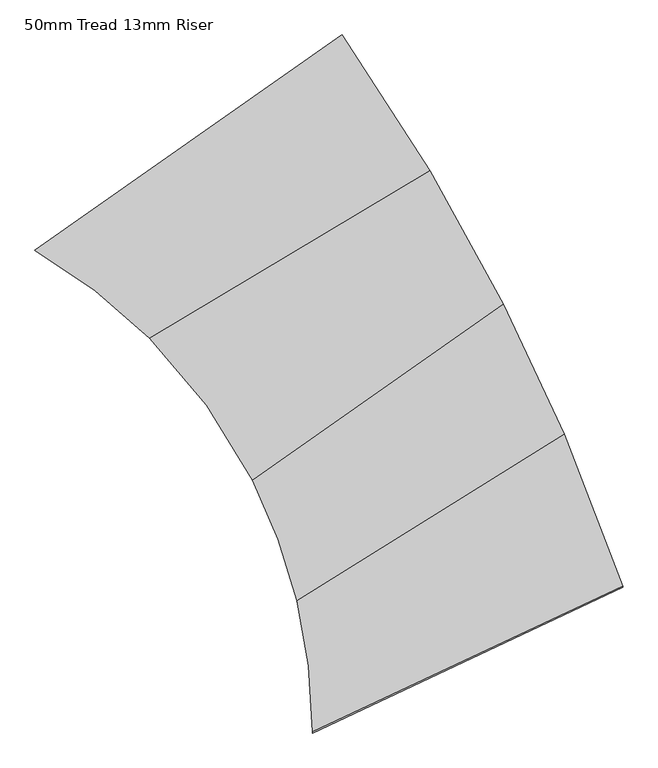
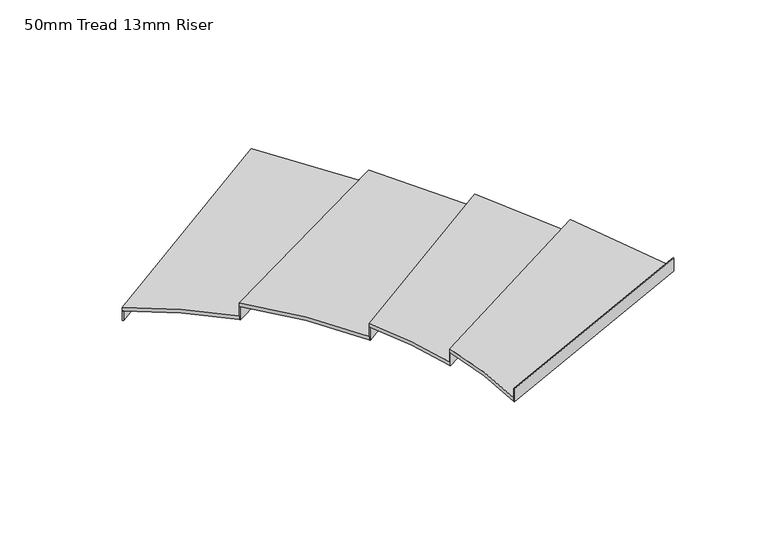
"""IFC4 building model written with IfcOpenShell, lengths in millimetres: stair flight geometry, 50mm Tread 13mm Riser."""

from ifc_helpers import new_model, si_unit, point, frame, frame_2d, origin, place, context, project, spatial, polyline, circle_curve, trimmed, segment, composite_curve, outline, extrude, source, transform, mapped, element, save


def stair_flight_50mm_tread_13mm_riser_794cdd2d(model_context):
    return source(origin(), model_context, "Body", "SweptSolid", [
        extrude(outline(composite_curve([segment(trimmed(circle_curve(frame_2d((18979.6163047, 39173.0351392)), 5303.3008589), [point((21646.6672, 43756.9024498))], [point((21634.7503997, 43763.8153492))], True, "CARTESIAN"), True, "CONTINUOUS"), segment(polyline([(21634.7503997, 43763.8153492), (24564.2523191, 45816.6486415)]), True, "CONTINUOUS"), segment(trimmed(circle_curve(frame_2d((7249.7804154, 33683.622161)), 21142.4045199), [point((24564.2523191, 45816.6486415))], [point((24571.4226886, 45806.4097053))], False, "CARTESIAN"), True, "CONTINUOUS"), segment(polyline([(24571.4226886, 45806.4097053), (21646.6672, 43756.9024498)]), True, "CONTINUOUS")], self_intersect=False)), frame((0.0, 0.0, 12000.0), z_axis=(0.0, 0.0, 1.0), x_axis=(1.0, 0.0, 0.0)), (0.0, 0.0, 1.0), 136.0465116),
        extrude(outline(composite_curve([segment(polyline([(25404.2827089, 44519.45694), (22729.6163047, 42923.0351392)]), True, "CONTINUOUS"), segment(trimmed(circle_curve(frame_2d((18979.6163047, 39173.0351392)), 5303.3008589), [point((22729.6163047, 42923.0351392))], [point((21634.7503997, 43763.8153492))], True, "CARTESIAN"), True, "CONTINUOUS"), segment(polyline([(21634.7503997, 43763.8153492), (24564.2523191, 45816.6486415)]), True, "CONTINUOUS"), segment(trimmed(circle_curve(frame_2d((7249.7804154, 33683.622161)), 21142.4045199), [point((24564.2523191, 45816.6486415))], [point((25404.2827089, 44519.45694))], False, "CARTESIAN"), True, "CONTINUOUS")], self_intersect=False)), frame((0.0, 0.0, 12136.0465116), z_axis=(0.0, 0.0, 1.0), x_axis=(1.0, 0.0, 0.0)), (0.0, 0.0, 1.0), 50.0),
        extrude(outline(composite_curve([segment(trimmed(circle_curve(frame_2d((18979.6163047, 39173.0351392)), 5303.3008589), [point((22738.7185782, 42913.910718))], [point((22729.6163047, 42923.0351392))], True, "CARTESIAN"), True, "CONTINUOUS"), segment(polyline([(22729.6163047, 42923.0351392), (25404.2827089, 44519.45694)]), True, "CONTINUOUS"), segment(trimmed(circle_curve(frame_2d((7249.7804154, 33683.622161)), 21142.4045199), [point((25404.2827089, 44519.45694))], [point((25410.6859943, 44508.7215803))], False, "CARTESIAN"), True, "CONTINUOUS"), segment(polyline([(25410.6859943, 44508.7215803), (22738.7185782, 42913.910718)]), True, "CONTINUOUS")], self_intersect=False)), frame((0.0, 0.0, 12136.0465116), z_axis=(0.0, 0.0, 1.0), x_axis=(1.0, 0.0, 0.0)), (0.0, 0.0, 1.0), 186.0465116),
        extrude(outline(composite_curve([segment(polyline([(26105.2845018, 43247.6816824), (23710.5359966, 41569.5740745)]), True, "CONTINUOUS"), segment(trimmed(circle_curve(frame_2d((18979.6163047, 39173.0351392)), 5303.3008589), [point((23710.5359966, 41569.5740745))], [point((22729.6163047, 42923.0351392))], True, "CARTESIAN"), True, "CONTINUOUS"), segment(polyline([(22729.6163047, 42923.0351392), (25404.2827089, 44519.45694)]), True, "CONTINUOUS"), segment(trimmed(circle_curve(frame_2d((7249.7804154, 33683.622161)), 21142.4045199), [point((25404.2827089, 44519.45694))], [point((26105.2845018, 43247.6816824))], False, "CARTESIAN"), True, "CONTINUOUS")], self_intersect=False)), frame((0.0, 0.0, 12322.0930233), z_axis=(0.0, 0.0, 1.0), x_axis=(1.0, 0.0, 0.0)), (0.0, 0.0, 1.0), 50.0),
        extrude(outline(composite_curve([segment(trimmed(circle_curve(frame_2d((18979.6163047, 39173.0351392)), 5303.3008589), [point((23716.2299584, 41558.3005532))], [point((23710.5359966, 41569.5740745))], True, "CARTESIAN"), True, "CONTINUOUS"), segment(polyline([(23710.5359966, 41569.5740745), (26105.2845018, 43247.6816824)]), True, "CONTINUOUS"), segment(trimmed(circle_curve(frame_2d((7249.7804154, 33683.622161)), 21142.4045199), [point((26105.2845018, 43247.6816824))], [point((26110.9932689, 43236.4185358))], False, "CARTESIAN"), True, "CONTINUOUS"), segment(polyline([(26110.9932689, 43236.4185358), (23716.2299584, 41558.3005532)]), True, "CONTINUOUS")], self_intersect=False)), frame((0.0, 0.0, 12322.0930233), z_axis=(0.0, 0.0, 1.0), x_axis=(1.0, 0.0, 0.0)), (0.0, 0.0, 1.0), 186.0465116),
        extrude(outline(composite_curve([segment(polyline([(26685.0925834, 42006.4768285), (24134.1926468, 40420.1689465)]), True, "CONTINUOUS"), segment(trimmed(circle_curve(frame_2d((18979.6163047, 39173.0351392)), 5303.3008589), [point((24134.1926468, 40420.1689465))], [point((23710.5359966, 41569.5740745))], True, "CARTESIAN"), True, "CONTINUOUS"), segment(polyline([(23710.5359966, 41569.5740745), (26105.2845018, 43247.6816824)]), True, "CONTINUOUS"), segment(trimmed(circle_curve(frame_2d((7249.7804154, 33683.622161)), 21142.4045199), [point((26105.2845018, 43247.6816824))], [point((26685.0925834, 42006.4768285))], False, "CARTESIAN"), True, "CONTINUOUS")], self_intersect=False)), frame((0.0, 0.0, 12508.1395349), z_axis=(0.0, 0.0, 1.0), x_axis=(1.0, 0.0, 0.0)), (0.0, 0.0, 1.0), 50.0),
        extrude(outline(composite_curve([segment(trimmed(circle_curve(frame_2d((18979.6163047, 39173.0351392)), 5303.3008589), [point((24137.2736797, 40407.3650796))], [point((24134.1926468, 40420.1689465))], True, "CARTESIAN"), True, "CONTINUOUS"), segment(polyline([(24134.1926468, 40420.1689465), (26685.0925834, 42006.4768285)]), True, "CONTINUOUS"), segment(trimmed(circle_curve(frame_2d((7249.7804154, 33683.622161)), 21142.4045199), [point((26685.0925834, 42006.4768285))], [point((26690.0672397, 41994.8505343))], False, "CARTESIAN"), True, "CONTINUOUS"), segment(polyline([(26690.0672397, 41994.8505343), (24137.2736797, 40407.3650796)]), True, "CONTINUOUS")], self_intersect=False)), frame((0.0, 0.0, 12508.1395349), z_axis=(0.0, 0.0, 1.0), x_axis=(1.0, 0.0, 0.0)), (0.0, 0.0, 1.0), 186.0465116),
        extrude(outline(composite_curve([segment(trimmed(circle_curve(frame_2d((18979.6163047, 39173.0351392)), 5303.3008589), [point((24282.8991769, 39159.2229355))], [point((24282.9171636, 39173.0351392))], True, "CARTESIAN"), True, "CONTINUOUS"), segment(polyline([(24282.9171636, 39173.0351392), (27242.7962676, 40559.7101488)]), True, "CONTINUOUS"), segment(trimmed(circle_curve(frame_2d((7249.7804154, 33683.622161)), 21142.4045199), [point((27242.7962676, 40559.7101488))], [point((27246.8815323, 40547.8202791))], False, "CARTESIAN"), True, "CONTINUOUS"), segment(polyline([(27246.8815323, 40547.8202791), (24282.8991769, 39159.2229355)]), True, "CONTINUOUS")], self_intersect=False)), frame((0.0, 0.0, 12694.1860465), z_axis=(0.0, 0.0, 1.0), x_axis=(1.0, 0.0, 0.0)), (0.0, 0.0, 1.0), 186.0465116),
        extrude(outline(composite_curve([segment(polyline([(27242.7962676, 40559.7101488), (24282.9171636, 39173.0351392)]), True, "CONTINUOUS"), segment(trimmed(circle_curve(frame_2d((18979.6163047, 39173.0351392)), 5303.3008589), [point((24282.9171636, 39173.0351392))], [point((24134.1926468, 40420.1689465))], True, "CARTESIAN"), True, "CONTINUOUS"), segment(polyline([(24134.1926468, 40420.1689465), (26685.0925834, 42006.4768285)]), True, "CONTINUOUS"), segment(trimmed(circle_curve(frame_2d((7249.7804154, 33683.622161)), 21142.4045199), [point((26685.0925834, 42006.4768285))], [point((27242.7962676, 40559.7101488))], False, "CARTESIAN"), True, "CONTINUOUS")], self_intersect=False)), frame((0.0, 0.0, 12694.1860465), z_axis=(0.0, 0.0, 1.0), x_axis=(1.0, 0.0, 0.0)), (0.0, 0.0, 1.0), 50.0),
    ])


if __name__ == "__main__":
    model = new_model("IFC4")
    model_context = context("Model", 3, world=origin())
    ifc_project = project(units=[si_unit("LENGTHUNIT", "METRE", prefix="MILLI")], contexts=[model_context])
    site = spatial("IfcSite", under=ifc_project)
    building = spatial("IfcBuilding", under=site)
    placement = place(None, origin())
    stair_flight_50mm_tread_13mm_riser_shape = stair_flight_50mm_tread_13mm_riser_794cdd2d(model_context)
    element("IfcStairFlight", 1, ObjectType="50mm Tread 13mm Riser", at=placement, inside=building, context=model_context, shape_type="MappedRepresentation", body=[
        mapped(stair_flight_50mm_tread_13mm_riser_shape, transform((0.0, 0.0, 0.0), x_axis=(1.0, 0.0, 0.0), y_axis=(0.0, 1.0, 0.0), z_axis=(0.0, 0.0, 1.0))),
    ])
    save(model, "model.ifc")
